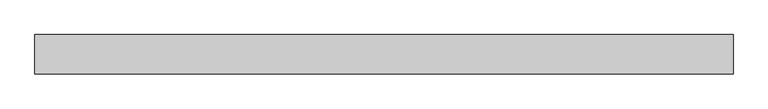
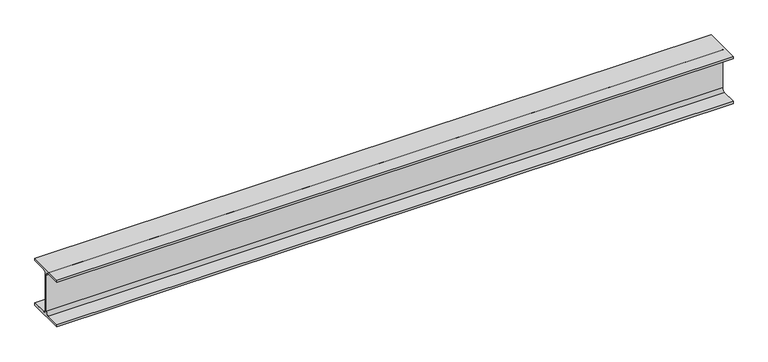
"""IFC4 building model written with IfcOpenShell, lengths in millimetres: beam geometry, 0912_Steel Framing_H-KSD3502 : H_SB_ASB_H-194x150x6x9."""

import ifcopenshell
import ifcopenshell.guid

model = None  # the IFC model being written
_history = None  # IfcOwnerHistory: only IFC2X3 demands one
_inside = {}  # id of a spatial element -> (the spatial element, [elements in it])
_under = {}  # id of a project, library or spatial element -> (it, [spatial elements below it])
_declared = {}  # id of a project -> (the project, [libraries it declares])
_typed = {}  # id of a type object -> (the type object, [elements of that type])
_made_of = {}  # id of a material, layer set ... -> (it, [elements and type objects made of it])


def new_model(schema):
    """Start an empty IFC model of exactly this schema.

    Asked for "IFC4X3", IfcOpenShell would pick the latest addendum, in which some entities
    have other attributes; the version numbers below select the first issue.
    IFC2X3 requires an IfcOwnerHistory on every rooted entity: one is made here for all.
    """
    global model, _history
    if schema == "IFC4X3":
        model = ifcopenshell.file(schema_version=(4, 3, 0, 0))
    else:
        model = ifcopenshell.file(schema=schema)
    _inside.clear()
    _under.clear()
    _declared.clear()
    _typed.clear()
    _made_of.clear()
    _history = None
    if model.schema == "IFC2X3":
        org = make("IfcOrganization", Name="unknown")
        user = make(
            "IfcPersonAndOrganization",
            ThePerson=make("IfcPerson", FamilyName="unknown"),
            TheOrganization=org,
        )
        app = make(
            "IfcApplication",
            ApplicationDeveloper=org,
            Version="unknown",
            ApplicationFullName="unknown",
            ApplicationIdentifier="unknown",
        )
        _history = make(
            "IfcOwnerHistory",
            OwningUser=user,
            OwningApplication=app,
            ChangeAction="ADDED",
            CreationDate=0,
        )
    return model


def make(cls, **values):
    """One entity of the class cls with the attributes given. An attribute that is None is left unset."""
    return model.create_entity(
        cls, **{name: value for name, value in values.items() if value is not None}
    )


def rooted(cls, **values):
    """An entity with a GlobalId (a new one), such as an element, a storey or a relation."""
    return make(cls, GlobalId=ifcopenshell.guid.new(), OwnerHistory=_history, **values)


def si_unit(unit_type, name, prefix=None):
    """IfcSIUnit, for example si_unit("LENGTHUNIT", "METRE", prefix="MILLI")."""
    return make("IfcSIUnit", UnitType=unit_type, Prefix=prefix, Name=name)


def assignment(units):
    """IfcUnitAssignment: the units of a project."""
    return None if units is None else make("IfcUnitAssignment", Units=units)


def point(xyz):
    """IfcCartesianPoint."""
    return None if xyz is None else make("IfcCartesianPoint", Coordinates=xyz)


def direction(xyz):
    """IfcDirection."""
    return None if xyz is None else make("IfcDirection", DirectionRatios=xyz)


def frame(location, z_axis=None, x_axis=None):
    """IfcAxis2Placement3D, a coordinate frame: its origin and axes. An axis left out is left unset."""
    return make(
        "IfcAxis2Placement3D",
        Location=point(location),
        Axis=direction(z_axis),
        RefDirection=direction(x_axis),
    )


def frame_2d(location, x_axis=None):
    """IfcAxis2Placement2D, a coordinate frame in the plane: its origin and x axis."""
    return make(
        "IfcAxis2Placement2D", Location=point(location), RefDirection=direction(x_axis)
    )


def origin():
    """The frame at (0, 0, 0) with its axes left unset."""
    return frame((0.0, 0.0, 0.0))


def place(relative_to, where):
    """IfcLocalPlacement: puts the frame where relative to a parent placement (None: the world)."""
    return make(
        "IfcLocalPlacement", PlacementRelTo=relative_to, RelativePlacement=where
    )


def context(
    kind, dimensions, precision=None, world=None, true_north=None, identifier=None
):
    """IfcGeometricRepresentationContext, for example the 3D "Model" context."""
    return make(
        "IfcGeometricRepresentationContext",
        ContextIdentifier=identifier,
        ContextType=kind,
        CoordinateSpaceDimension=dimensions,
        Precision=precision,
        WorldCoordinateSystem=world,
        TrueNorth=true_north,
    )


def project(units=None, contexts=None):
    """IfcProject with its units and contexts."""
    return rooted(
        "IfcProject",
        Name="project",
        RepresentationContexts=contexts,
        UnitsInContext=assignment(units),
    )


def spatial(cls, under=None, at=None, **own):
    """A site, building, storey or space (cls), placed at a placement, below another one or the project."""
    s = rooted(cls, ObjectPlacement=at, **own)
    if under is not None:
        _under.setdefault(under.id(), (under, []))[1].append(s)
    return s


def polyline(points):
    """IfcPolyline through the points."""
    return make("IfcPolyline", Points=[point(p) for p in points])


def circle_curve(where, radius):
    """IfcCircle in the frame where."""
    return make("IfcCircle", Position=where, Radius=radius)


def trimmed(basis, trim1, trim2, sense, master):
    """IfcTrimmedCurve: the piece of a basis curve between two trims."""
    return make(
        "IfcTrimmedCurve",
        BasisCurve=basis,
        Trim1=trim1,
        Trim2=trim2,
        SenseAgreement=sense,
        MasterRepresentation=master,
    )


def segment(curve, same_sense, transition):
    """IfcCompositeCurveSegment."""
    return make(
        "IfcCompositeCurveSegment",
        Transition=transition,
        SameSense=same_sense,
        ParentCurve=curve,
    )


def composite_curve(segments, self_intersect=None):
    """IfcCompositeCurve: segments joined end to end."""
    return make("IfcCompositeCurve", Segments=segments, SelfIntersect=self_intersect)


def outline(outer, holes=None, kind="AREA"):
    """IfcArbitraryClosedProfileDef: a profile drawn as a closed curve; with holes, ...WithVoids."""
    if holes is None:
        return make("IfcArbitraryClosedProfileDef", ProfileType=kind, OuterCurve=outer)
    return make(
        "IfcArbitraryProfileDefWithVoids",
        ProfileType=kind,
        OuterCurve=outer,
        InnerCurves=holes,
    )


def extrude(swept, where, along, depth):
    """IfcExtrudedAreaSolid: the profile swept, set in the frame where, extruded along a direction by depth."""
    return make(
        "IfcExtrudedAreaSolid",
        SweptArea=swept,
        Position=where,
        ExtrudedDirection=direction(along),
        Depth=depth,
    )


def shape(context_of_items, identifier, shape_type, items):
    """IfcShapeRepresentation: the items that make up one representation, for example the "Body"."""
    return make(
        "IfcShapeRepresentation",
        ContextOfItems=context_of_items,
        RepresentationIdentifier=identifier,
        RepresentationType=shape_type,
        Items=items,
    )


def source(mapping_origin, context_of_items, identifier, shape_type, items):
    """IfcRepresentationMap: a shape defined once, which mapped items show again and again."""
    return make(
        "IfcRepresentationMap",
        MappingOrigin=mapping_origin,
        MappedRepresentation=shape(context_of_items, identifier, shape_type, items),
    )


def transform(
    local_origin,
    x_axis=None,
    y_axis=None,
    z_axis=None,
    scale=None,
    scale2=None,
    scale3=None,
    uniform=True,
):
    """IfcCartesianTransformationOperator3D, or its non-uniform kind. x_axis, y_axis, z_axis: its Axis1, 2, 3."""
    if uniform:
        return make(
            "IfcCartesianTransformationOperator3D",
            Axis1=direction(x_axis),
            Axis2=direction(y_axis),
            LocalOrigin=point(local_origin),
            Scale=scale,
            Axis3=direction(z_axis),
        )
    return make(
        "IfcCartesianTransformationOperator3DnonUniform",
        Axis1=direction(x_axis),
        Axis2=direction(y_axis),
        LocalOrigin=point(local_origin),
        Scale=scale,
        Axis3=direction(z_axis),
        Scale2=scale2,
        Scale3=scale3,
    )


def mapped(mapping_source, mapping_target):
    """IfcMappedItem: shows the shape of a source again, moved by a transform."""
    return make(
        "IfcMappedItem", MappingSource=mapping_source, MappingTarget=mapping_target
    )


def made_of(thing, what):
    """Note that an element or type object is made of a material, layer set ...; save() writes the relation."""
    if what is not None:
        _made_of.setdefault(what.id(), (what, []))[1].append(thing)
    return thing


def element(
    cls,
    number,
    at=None,
    inside=None,
    cuts=None,
    type_object=None,
    material=None,
    context=None,
    identifier="Body",
    shape_type=None,
    held_by="IfcProductDefinitionShape",
    body=None,
    shapes=None,
    **own,
):
    """One element of the class cls, such as IfcWall. Its Tag is "e" and its number.

    at: its placement. inside: the storey or other place that contains it. cuts: it is an
    opening in that element (IfcRelVoidsElement). A single representation is given by context,
    identifier, shape_type and body (its items); several are given by shapes. held_by: the class
    of the entity that holds the representations. save() writes the other relations.
    """
    e = rooted(cls, Tag="e%d" % number, ObjectPlacement=at, **own)
    if body is not None:
        shapes = [shape(context, identifier, shape_type, body)]
    if shapes is not None:
        e.Representation = make(held_by, Representations=shapes)
    if inside is not None:
        _inside.setdefault(inside.id(), (inside, []))[1].append(e)
    if cuts is not None:
        rooted(
            "IfcRelVoidsElement", RelatingBuildingElement=cuts, RelatedOpeningElement=e
        )
    if type_object is not None:
        _typed.setdefault(type_object.id(), (type_object, []))[1].append(e)
    return made_of(e, material)


def aggregate(whole, parts):
    """IfcRelAggregates: a whole, such as a stair, and the parts it consists of."""
    return rooted("IfcRelAggregates", RelatingObject=whole, RelatedObjects=parts)


def save(model, path):
    """Write the relations noted so far, then the file.

    IfcRelAggregates (storeys below a building ...), IfcRelContainedInSpatialStructure (elements
    in a storey), IfcRelDefinesByType, IfcRelAssociatesMaterial and IfcRelDeclares: one each for
    every whole, place, type object, material and project.
    """
    for whole, parts in _under.values():
        aggregate(whole, parts)
    for where, things in _inside.values():
        rooted(
            "IfcRelContainedInSpatialStructure",
            RelatedElements=things,
            RelatingStructure=where,
        )
    for kind, things in _typed.values():
        rooted("IfcRelDefinesByType", RelatedObjects=things, RelatingType=kind)
    for what, things in _made_of.values():
        rooted("IfcRelAssociatesMaterial", RelatedObjects=things, RelatingMaterial=what)
    for by, libraries in _declared.values():
        rooted("IfcRelDeclares", RelatingContext=by, RelatedDefinitions=libraries)
    model.write(path)


def beam_978064fb(model_context):
    return source(origin(), model_context, "Body", "SweptSolid", [
        extrude(outline(composite_curve([segment(polyline([(-75.0, -88.0), (-16.0, -88.0)]), True, "CONTINUOUS"), segment(trimmed(circle_curve(frame_2d((-16.0, -75.0)), 13.0), [point((-16.0, -88.0))], [point((-3.0, -75.0))], True, "CARTESIAN"), True, "CONTINUOUS"), segment(polyline([(-3.0, -75.0), (-3.0, 75.0)]), True, "CONTINUOUS"), segment(trimmed(circle_curve(frame_2d((-16.0, 75.0)), 13.0), [point((-3.0, 75.0))], [point((-16.0, 88.0))], True, "CARTESIAN"), True, "CONTINUOUS"), segment(polyline([(-16.0, 88.0), (-75.0, 88.0), (-75.0, 97.0), (75.0, 97.0), (75.0, 88.0), (16.0, 88.0)]), True, "CONTINUOUS"), segment(trimmed(circle_curve(frame_2d((16.0, 75.0)), 13.0), [point((16.0, 88.0))], [point((3.0, 75.0))], True, "CARTESIAN"), True, "CONTINUOUS"), segment(polyline([(3.0, 75.0), (3.0, -75.0)]), True, "CONTINUOUS"), segment(trimmed(circle_curve(frame_2d((16.0, -75.0)), 13.0), [point((3.0, -75.0))], [point((16.0, -88.0))], True, "CARTESIAN"), True, "CONTINUOUS"), segment(polyline([(16.0, -88.0), (75.0, -88.0), (75.0, -97.0), (-75.0, -97.0), (-75.0, -88.0)]), True, "CONTINUOUS")], self_intersect=False)), frame((-1106.6961534, 0.0, 0.0), z_axis=(1.0, 0.0, 0.0), x_axis=(0.0, 1.0, 0.0)), (0.0, 0.0, 1.0), 2655.7235444),
    ])


if __name__ == "__main__":
    model = new_model("IFC4")
    model_context = context("Model", 3, world=origin())
    ifc_project = project(units=[si_unit("LENGTHUNIT", "METRE", prefix="MILLI")], contexts=[model_context])
    site = spatial("IfcSite", under=ifc_project)
    building = spatial("IfcBuilding", under=site)
    placement = place(None, origin())
    beam_shape = beam_978064fb(model_context)
    element("IfcBeam", 1, ObjectType="0912_Steel Framing_H-KSD3502 : H_SB_ASB_H-194x150x6x9", at=placement, inside=building, context=model_context, shape_type="MappedRepresentation", body=[
        mapped(beam_shape, transform((0.0, 0.0, 0.0), x_axis=(1.0, 0.0, 0.0), y_axis=(0.0, 1.0, 0.0), z_axis=(0.0, 0.0, 1.0))),
    ])
    save(model, "model.ifc")

# Revit data of these elements
# Type "0912_Steel Framing_H-KSD3502 : H_SB_ASB_H-194x150x6x9"
#   H_WM Code_1 = "S01AA002-00001 | Main Steel Structure Fabrication Work | Shelter/Building | Medium Steel - Standard (90KG/M>Weight≥30KG/M) | Material: (   )"
#   H_WM Code_2 = "S03AA028-00001 | Main Steel Structure Erection Work | Shelter/Building | Medium Steel (90KG/M>Weight≥30KG/M) | Material: (   )"
#   H_WM Code_3 = "S01AA010-00001 | Main Steel Structure Fabrication Work | Shelter/Building | Steel Painting/Coating | for Non-Fireproofed Steel Surface, Surface Preparation, Primer, Second & Final Coat | Material: (   )"
#   H_Q'ty Cal Type Tag = "SB-Q2"
#   Width = 15.0 cm
#   Web Thickness = 0.6 cm
#   Web Fillet = 1.3 cm
#   Warping Constant = 43316.0 cm⁶
#   W = 0
#   Torsional Moment of Inertia = 8.622 cm⁴
#   Section Area = 39.01 cm²
#   Plastic Modulus weak axis = 104.0 cm³
#   Plastic Modulus strong axis = 309.0 cm³
#   Perimeter = 0.95 m²/m
#   Nominal Weight = 30.60 kgf/m
#   Moment of Inertia weak axis = 507.00 cm⁴
#   Moment of Inertia strong axis = 2690.00 cm⁴
#   Height = 19.4 cm
#   Flange Thickness = 0.9 cm
#   Elastic Modulus weak axis = 67.6 cm³
#   Elastic Modulus strong axis = 277.0 cm³
#   Centroid Vertical = 9.7 cm
#   Centroid Horizontal = 7.5 cm
#   Ix = 26900000
#   Length [instance default] = 1.5240 m
#   Zx = 309000
#   b = 0.1500 m
#   h = 0.1940 m
#   r = 0.0130 m
#   s = 0.0060 m
#   t = 0.0090 m
#   A = 0.003901 m²
#   Structural Material [instance default] = Steel, 45-345
#   Assembly Code = ""
# Element 1 (IfcBeam, "0912_Steel Framing_H-KSD3502 : H_SB_ASB_H-194x150x6x9")
#   Structural Material = none
# Materials
#   "Steel, 45-345": class "Metal", colour RGB 189 187 185, transparency 0, Description = "Steel 345 MPa", Cost = 0
